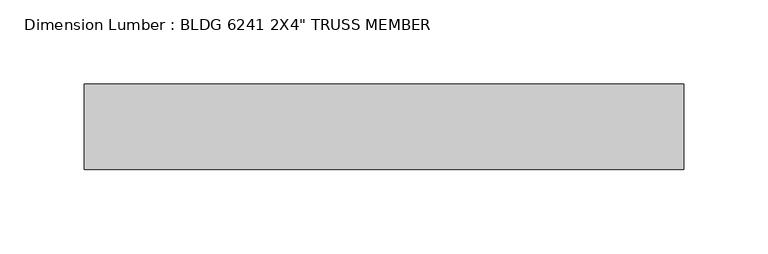
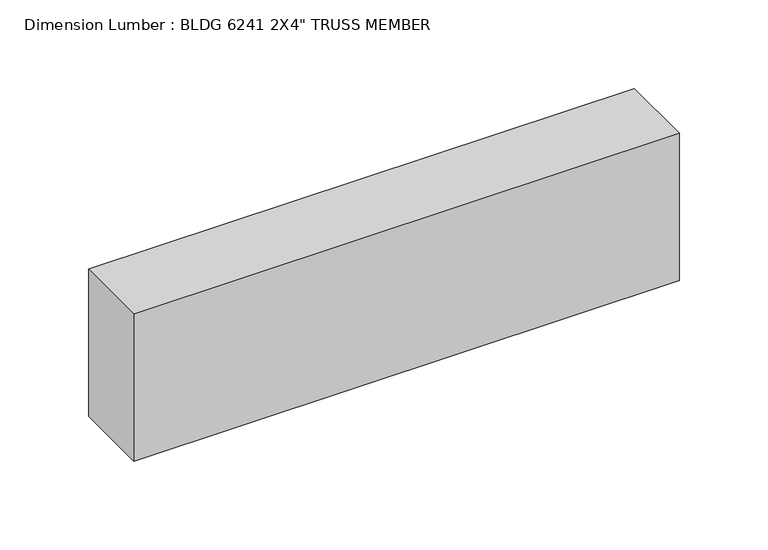
"""IFC4 building model written with IfcOpenShell, lengths in millimetres: beam geometry."""

import ifcopenshell
import ifcopenshell.guid

model = None  # the IFC model being written
_history = None  # IfcOwnerHistory: only IFC2X3 demands one
_inside = {}  # id of a spatial element -> (the spatial element, [elements in it])
_under = {}  # id of a project, library or spatial element -> (it, [spatial elements below it])
_declared = {}  # id of a project -> (the project, [libraries it declares])
_typed = {}  # id of a type object -> (the type object, [elements of that type])
_made_of = {}  # id of a material, layer set ... -> (it, [elements and type objects made of it])


def new_model(schema):
    """Start an empty IFC model of exactly this schema.

    Asked for "IFC4X3", IfcOpenShell would pick the latest addendum, in which some entities
    have other attributes; the version numbers below select the first issue.
    IFC2X3 requires an IfcOwnerHistory on every rooted entity: one is made here for all.
    """
    global model, _history
    if schema == "IFC4X3":
        model = ifcopenshell.file(schema_version=(4, 3, 0, 0))
    else:
        model = ifcopenshell.file(schema=schema)
    _inside.clear()
    _under.clear()
    _declared.clear()
    _typed.clear()
    _made_of.clear()
    _history = None
    if model.schema == "IFC2X3":
        org = make("IfcOrganization", Name="unknown")
        user = make(
            "IfcPersonAndOrganization",
            ThePerson=make("IfcPerson", FamilyName="unknown"),
            TheOrganization=org,
        )
        app = make(
            "IfcApplication",
            ApplicationDeveloper=org,
            Version="unknown",
            ApplicationFullName="unknown",
            ApplicationIdentifier="unknown",
        )
        _history = make(
            "IfcOwnerHistory",
            OwningUser=user,
            OwningApplication=app,
            ChangeAction="ADDED",
            CreationDate=0,
        )
    return model


def make(cls, **values):
    """One entity of the class cls with the attributes given. An attribute that is None is left unset."""
    return model.create_entity(
        cls, **{name: value for name, value in values.items() if value is not None}
    )


def rooted(cls, **values):
    """An entity with a GlobalId (a new one), such as an element, a storey or a relation."""
    return make(cls, GlobalId=ifcopenshell.guid.new(), OwnerHistory=_history, **values)


def si_unit(unit_type, name, prefix=None):
    """IfcSIUnit, for example si_unit("LENGTHUNIT", "METRE", prefix="MILLI")."""
    return make("IfcSIUnit", UnitType=unit_type, Prefix=prefix, Name=name)


def assignment(units):
    """IfcUnitAssignment: the units of a project."""
    return None if units is None else make("IfcUnitAssignment", Units=units)


def point(xyz):
    """IfcCartesianPoint."""
    return None if xyz is None else make("IfcCartesianPoint", Coordinates=xyz)


def direction(xyz):
    """IfcDirection."""
    return None if xyz is None else make("IfcDirection", DirectionRatios=xyz)


def frame(location, z_axis=None, x_axis=None):
    """IfcAxis2Placement3D, a coordinate frame: its origin and axes. An axis left out is left unset."""
    return make(
        "IfcAxis2Placement3D",
        Location=point(location),
        Axis=direction(z_axis),
        RefDirection=direction(x_axis),
    )


def origin():
    """The frame at (0, 0, 0) with its axes left unset."""
    return frame((0.0, 0.0, 0.0))


def place(relative_to, where):
    """IfcLocalPlacement: puts the frame where relative to a parent placement (None: the world)."""
    return make(
        "IfcLocalPlacement", PlacementRelTo=relative_to, RelativePlacement=where
    )


def context(
    kind, dimensions, precision=None, world=None, true_north=None, identifier=None
):
    """IfcGeometricRepresentationContext, for example the 3D "Model" context."""
    return make(
        "IfcGeometricRepresentationContext",
        ContextIdentifier=identifier,
        ContextType=kind,
        CoordinateSpaceDimension=dimensions,
        Precision=precision,
        WorldCoordinateSystem=world,
        TrueNorth=true_north,
    )


def project(units=None, contexts=None):
    """IfcProject with its units and contexts."""
    return rooted(
        "IfcProject",
        Name="project",
        RepresentationContexts=contexts,
        UnitsInContext=assignment(units),
    )


def spatial(cls, under=None, at=None, **own):
    """A site, building, storey or space (cls), placed at a placement, below another one or the project."""
    s = rooted(cls, ObjectPlacement=at, **own)
    if under is not None:
        _under.setdefault(under.id(), (under, []))[1].append(s)
    return s


def polyline(points):
    """IfcPolyline through the points."""
    return make("IfcPolyline", Points=[point(p) for p in points])


def outline(outer, holes=None, kind="AREA"):
    """IfcArbitraryClosedProfileDef: a profile drawn as a closed curve; with holes, ...WithVoids."""
    if holes is None:
        return make("IfcArbitraryClosedProfileDef", ProfileType=kind, OuterCurve=outer)
    return make(
        "IfcArbitraryProfileDefWithVoids",
        ProfileType=kind,
        OuterCurve=outer,
        InnerCurves=holes,
    )


def extrude(swept, where, along, depth):
    """IfcExtrudedAreaSolid: the profile swept, set in the frame where, extruded along a direction by depth."""
    return make(
        "IfcExtrudedAreaSolid",
        SweptArea=swept,
        Position=where,
        ExtrudedDirection=direction(along),
        Depth=depth,
    )


def shape(context_of_items, identifier, shape_type, items):
    """IfcShapeRepresentation: the items that make up one representation, for example the "Body"."""
    return make(
        "IfcShapeRepresentation",
        ContextOfItems=context_of_items,
        RepresentationIdentifier=identifier,
        RepresentationType=shape_type,
        Items=items,
    )


def source(mapping_origin, context_of_items, identifier, shape_type, items):
    """IfcRepresentationMap: a shape defined once, which mapped items show again and again."""
    return make(
        "IfcRepresentationMap",
        MappingOrigin=mapping_origin,
        MappedRepresentation=shape(context_of_items, identifier, shape_type, items),
    )


def transform(
    local_origin,
    x_axis=None,
    y_axis=None,
    z_axis=None,
    scale=None,
    scale2=None,
    scale3=None,
    uniform=True,
):
    """IfcCartesianTransformationOperator3D, or its non-uniform kind. x_axis, y_axis, z_axis: its Axis1, 2, 3."""
    if uniform:
        return make(
            "IfcCartesianTransformationOperator3D",
            Axis1=direction(x_axis),
            Axis2=direction(y_axis),
            LocalOrigin=point(local_origin),
            Scale=scale,
            Axis3=direction(z_axis),
        )
    return make(
        "IfcCartesianTransformationOperator3DnonUniform",
        Axis1=direction(x_axis),
        Axis2=direction(y_axis),
        LocalOrigin=point(local_origin),
        Scale=scale,
        Axis3=direction(z_axis),
        Scale2=scale2,
        Scale3=scale3,
    )


def mapped(mapping_source, mapping_target):
    """IfcMappedItem: shows the shape of a source again, moved by a transform."""
    return make(
        "IfcMappedItem", MappingSource=mapping_source, MappingTarget=mapping_target
    )


def made_of(thing, what):
    """Note that an element or type object is made of a material, layer set ...; save() writes the relation."""
    if what is not None:
        _made_of.setdefault(what.id(), (what, []))[1].append(thing)
    return thing


def element(
    cls,
    number,
    at=None,
    inside=None,
    cuts=None,
    type_object=None,
    material=None,
    context=None,
    identifier="Body",
    shape_type=None,
    held_by="IfcProductDefinitionShape",
    body=None,
    shapes=None,
    **own,
):
    """One element of the class cls, such as IfcWall. Its Tag is "e" and its number.

    at: its placement. inside: the storey or other place that contains it. cuts: it is an
    opening in that element (IfcRelVoidsElement). A single representation is given by context,
    identifier, shape_type and body (its items); several are given by shapes. held_by: the class
    of the entity that holds the representations. save() writes the other relations.
    """
    e = rooted(cls, Tag="e%d" % number, ObjectPlacement=at, **own)
    if body is not None:
        shapes = [shape(context, identifier, shape_type, body)]
    if shapes is not None:
        e.Representation = make(held_by, Representations=shapes)
    if inside is not None:
        _inside.setdefault(inside.id(), (inside, []))[1].append(e)
    if cuts is not None:
        rooted(
            "IfcRelVoidsElement", RelatingBuildingElement=cuts, RelatedOpeningElement=e
        )
    if type_object is not None:
        _typed.setdefault(type_object.id(), (type_object, []))[1].append(e)
    return made_of(e, material)


def aggregate(whole, parts):
    """IfcRelAggregates: a whole, such as a stair, and the parts it consists of."""
    return rooted("IfcRelAggregates", RelatingObject=whole, RelatedObjects=parts)


def save(model, path):
    """Write the relations noted so far, then the file.

    IfcRelAggregates (storeys below a building ...), IfcRelContainedInSpatialStructure (elements
    in a storey), IfcRelDefinesByType, IfcRelAssociatesMaterial and IfcRelDeclares: one each for
    every whole, place, type object, material and project.
    """
    for whole, parts in _under.values():
        aggregate(whole, parts)
    for where, things in _inside.values():
        rooted(
            "IfcRelContainedInSpatialStructure",
            RelatedElements=things,
            RelatingStructure=where,
        )
    for kind, things in _typed.values():
        rooted("IfcRelDefinesByType", RelatedObjects=things, RelatingType=kind)
    for what, things in _made_of.values():
        rooted("IfcRelAssociatesMaterial", RelatedObjects=things, RelatingMaterial=what)
    for by, libraries in _declared.values():
        rooted("IfcRelDeclares", RelatingContext=by, RelatedDefinitions=libraries)
    model.write(path)


def beam_7aad778a(model_context):
    return source(origin(), model_context, "Body", "SweptSolid", [
        extrude(outline(polyline([(307.975, -25.4), (-47.625, -25.4), (-47.625, 25.4), (307.975, 25.4), (307.975, -25.4)])), frame((0.0, 0.0, -50.8), z_axis=(0.0, 0.0, 1.0), x_axis=(1.0, 0.0, 0.0)), (0.0, 0.0, 1.0), 101.6),
    ])


if __name__ == "__main__":
    model = new_model("IFC4")
    model_context = context("Model", 3, world=origin())
    ifc_project = project(units=[si_unit("LENGTHUNIT", "METRE", prefix="MILLI")], contexts=[model_context])
    site = spatial("IfcSite", under=ifc_project)
    building = spatial("IfcBuilding", under=site)
    placement = place(None, origin())
    beam_shape = beam_7aad778a(model_context)
    element("IfcBeam", 1, ObjectType="Dimension Lumber : BLDG 6241 2X4\" TRUSS MEMBER", at=placement, inside=building, context=model_context, shape_type="MappedRepresentation", body=[
        mapped(beam_shape, transform((0.0, 0.0, 0.0), x_axis=(1.0, 0.0, 0.0), y_axis=(0.0, 1.0, 0.0), z_axis=(0.0, 0.0, 1.0))),
    ])
    save(model, "model.ifc")

# Revit data of these elements
# Type "Dimension Lumber : BLDG 6241 2X4\" TRUSS MEMBER"
#   Assembly Code = "B10"
#   A = 0.273472 SF
#   Length [instance default] = 5' - 0"
#   b = 0' - 2"
#   d = 0' - 4"
#   Structural Material [instance default] = Softwood, Lumber
# Element 1 (IfcBeam, "Dimension Lumber : BLDG 6241 2X4\" TRUSS MEMBER")
#   Materials on its faces: "Softwood, Lumber"
# Materials
#   "Softwood, Lumber": class "Wood", colour RGB 223 192 134, transparency 0, Description = "Pinus Echinata", Cost = 0
